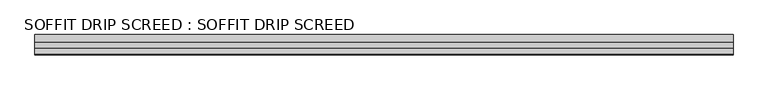
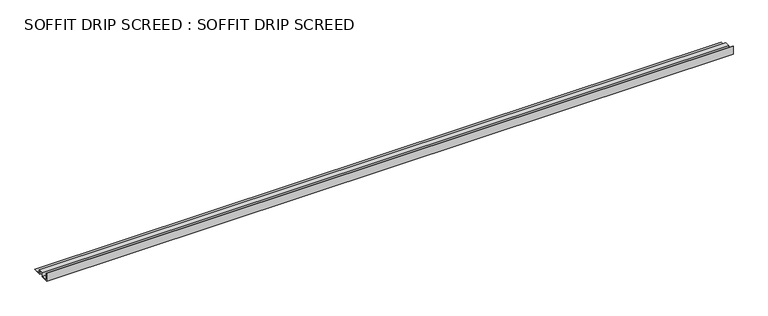
"""IFC4 building model written with IfcOpenShell, lengths in millimetres: proxy geometry, SOFFIT DRIP SCREED : SOFFIT DRIP SCREED."""

from ifc_helpers import new_model, si_unit, frame, origin, place, context, project, spatial, polyline, outline, extrude, source, transform, mapped, element, save


def soffit_drip_screed_soffit_drip_screed_06f9d920(model_context):
    return source(origin(), model_context, "Body", "SweptSolid", [
        extrude(outline(polyline([(-5503.7598427, 39712.8039618), (-5527.4730267, 39712.8039618), (-5527.4730267, 39724.2339618), (-5540.1730267, 39724.2339618), (-5540.1730267, 39712.8039618), (-5562.3980267, 39712.8039618), (-5562.3980267, 39736.6047233), (-5561.1180267, 39736.6047233), (-5561.1180267, 39714.0839618), (-5541.4530267, 39714.0839618), (-5541.4530267, 39725.5139618), (-5526.1930267, 39725.5139618), (-5526.1930267, 39714.0839618), (-5503.7598427, 39714.0839618), (-5503.7598427, 39712.8039618)])), frame((12382.7678845, 0.0, 0.0), z_axis=(1.0, 0.0, 0.0), x_axis=(0.0, 1.0, 0.0)), (0.0, 0.0, 1.0), 2000.25),
    ])


if __name__ == "__main__":
    model = new_model("IFC4")
    model_context = context("Model", 3, world=origin())
    ifc_project = project(units=[si_unit("LENGTHUNIT", "METRE", prefix="MILLI")], contexts=[model_context])
    site = spatial("IfcSite", under=ifc_project)
    building = spatial("IfcBuilding", under=site)
    placement = place(None, origin())
    soffit_drip_screed_soffit_drip_screed_shape = soffit_drip_screed_soffit_drip_screed_06f9d920(model_context)
    element("IfcBuildingElementProxy", 1, Name="SOFFIT DRIP SCREED : SOFFIT DRIP SCREED", ObjectType="SOFFIT DRIP SCREED : SOFFIT DRIP SCREED", at=placement, inside=building, context=model_context, shape_type="MappedRepresentation", body=[
        mapped(soffit_drip_screed_soffit_drip_screed_shape, transform((0.0, 0.0, 0.0), x_axis=(1.0, 0.0, 0.0), y_axis=(0.0, 1.0, 0.0), z_axis=(0.0, 0.0, 1.0))),
    ])
    save(model, "model.ifc")

# Revit data of these elements
# Type "SOFFIT DRIP SCREED : SOFFIT DRIP SCREED"
#   NameOverride = "SOFFIT DRIP SCREED"
# Element 1 (IfcBuildingElementProxy, "SOFFIT DRIP SCREED : SOFFIT DRIP SCREED")
#   Materials on its faces: "16 GA. COPPER VENTED SOFFIT DRIP SCREED"
# Materials
#   "16 GA. COPPER VENTED SOFFIT DRIP SCREED": class "Unassigned", colour RGB 85 255 127, transparency 0
